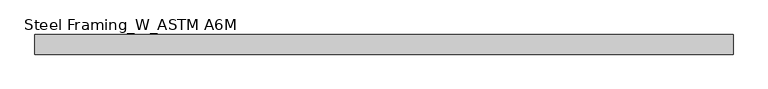
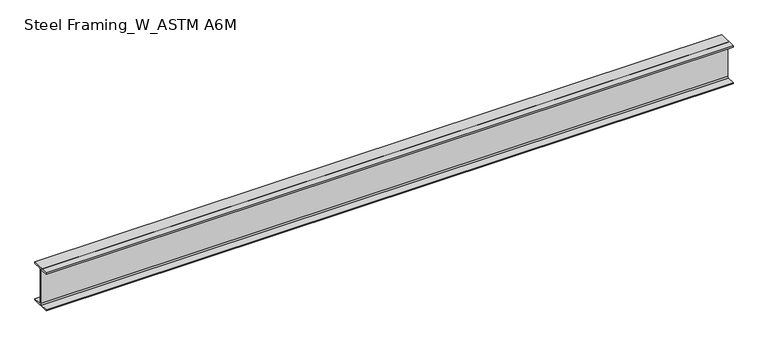
"""IFC4 building model written with IfcOpenShell, lengths in millimetres: beam geometry, Steel Framing_W_ASTM A6M : H_SB_AR_S02_W360x51_RG1."""

from ifc_helpers import new_model, si_unit, point, frame, frame_2d, origin, place, context, project, spatial, polyline, circle_curve, trimmed, segment, composite_curve, outline, extrude, source, transform, mapped, element, save


def steel_framing_w_astm_a6m_067f4f2a(model_context):
    return source(origin(), model_context, "Body", "SweptSolid", [
        extrude(outline(composite_curve([segment(polyline([(85.5, -166.4), (85.5, -178.0), (-85.5, -178.0), (-85.5, -166.4), (-13.72, -166.4)]), True, "CONTINUOUS"), segment(trimmed(circle_curve(frame_2d((-13.72, -156.3)), 10.1), [point((-13.72, -166.4))], [point((-3.62, -156.3))], True, "CARTESIAN"), True, "CONTINUOUS"), segment(polyline([(-3.62, -156.3), (-3.62, 156.3)]), True, "CONTINUOUS"), segment(trimmed(circle_curve(frame_2d((-13.72, 156.3)), 10.1), [point((-3.62, 156.3))], [point((-13.72, 166.4))], True, "CARTESIAN"), True, "CONTINUOUS"), segment(polyline([(-13.72, 166.4), (-85.5, 166.4), (-85.5, 178.0), (85.5, 178.0), (85.5, 166.4), (13.72, 166.4)]), True, "CONTINUOUS"), segment(trimmed(circle_curve(frame_2d((13.72, 156.3)), 10.1), [point((13.72, 166.4))], [point((3.62, 156.3))], True, "CARTESIAN"), True, "CONTINUOUS"), segment(polyline([(3.62, 156.3), (3.62, -156.3)]), True, "CONTINUOUS"), segment(trimmed(circle_curve(frame_2d((13.72, -156.3)), 10.1), [point((3.62, -156.3))], [point((13.72, -166.4))], True, "CARTESIAN"), True, "CONTINUOUS"), segment(polyline([(13.72, -166.4), (85.5, -166.4)]), True, "CONTINUOUS")], self_intersect=False)), frame((-3045.45, 0.0, 0.0), z_axis=(1.0, 0.0, 0.0), x_axis=(0.0, 1.0, 0.0)), (0.0, 0.0, 1.0), 6090.9),
    ])


if __name__ == "__main__":
    model = new_model("IFC4")
    model_context = context("Model", 3, world=origin())
    ifc_project = project(units=[si_unit("LENGTHUNIT", "METRE", prefix="MILLI")], contexts=[model_context])
    site = spatial("IfcSite", under=ifc_project)
    building = spatial("IfcBuilding", under=site)
    placement = place(None, origin())
    steel_framing_w_astm_a6m_shape = steel_framing_w_astm_a6m_067f4f2a(model_context)
    element("IfcBeam", 1, ObjectType="Steel Framing_W_ASTM A6M : H_SB_AR_S02_W360x51_RG1", at=placement, inside=building, context=model_context, shape_type="MappedRepresentation", body=[
        mapped(steel_framing_w_astm_a6m_shape, transform((0.0, 0.0, 0.0), x_axis=(1.0, 0.0, 0.0), y_axis=(0.0, 1.0, 0.0), z_axis=(0.0, 0.0, 1.0))),
    ])
    save(model, "model.ifc")

# Revit data of these elements
# Type "Steel Framing_W_ASTM A6M : H_SB_AR_S02_W360x51_RG1"
#   Type Mark = "RG1"
#   Section Name Key = "W14x34"
#   Width = 17.1 cm
#   Web Thickness = 0.724 cm
#   Web Fillet = 1.01 cm
#   Warping Constant = 287000.0 cm⁶
#   Torsional Moment of Inertia = 23.70 cm⁴
#   Section Area = 64.5 cm²
#   Plastic Modulus weak axis = 174.0 cm³
#   Plastic Modulus strong axis = 895.0 cm³
#   Perimeter = 1.36 m²/m
#   Nominal Weight = 51.00 kgf/m
#   Moment of Inertia weak axis = 970.00 cm⁴
#   Moment of Inertia strong axis = 14200.00 cm⁴
#   Height = 35.6 cm
#   Flange Thickness = 1.16 cm
#   Elastic Modulus weak axis = 113.0 cm³
#   Elastic Modulus strong axis = 796.0 cm³
#   Centroid Vertical = 17.8 cm
#   Centroid Horizontal = 8.55 cm
#   Length [instance default] = 1500 mm
#   Structural Material [instance default] = Steel, 45-345
#   Bolt Spacing = 0
#   Assembly Code = ""
# Element 1 (IfcBeam, "Steel Framing_W_ASTM A6M : H_SB_AR_S02_W360x51_RG1")
#   Materials on its faces: "Steel, 45-345"
# Materials
#   "Steel, 45-345": class "Metal", colour RGB 189 187 185, transparency 0, Description = "Steel 345 MPa", Cost = 0
